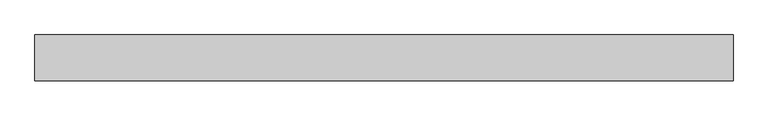
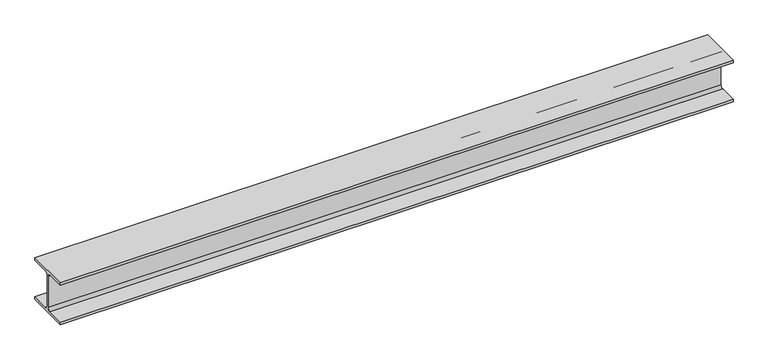
"""IFC4 building model written with IfcOpenShell, lengths in millimetres: beam geometry, 0912_Steel Framing_H-KSD3502 : H_SB_ASB_H-200x200x8x12."""

from ifc_helpers import new_model, si_unit, point, frame, frame_2d, origin, place, context, project, spatial, polyline, circle_curve, trimmed, segment, composite_curve, outline, extrude, source, transform, mapped, element, save


def beam_a4cbd311(model_context):
    return source(origin(), model_context, "Body", "SweptSolid", [
        extrude(outline(composite_curve([segment(polyline([(100.0, -88.0), (100.0, -100.0), (-100.0, -100.0), (-100.0, -88.0), (-17.0, -88.0)]), True, "CONTINUOUS"), segment(trimmed(circle_curve(frame_2d((-17.0, -75.0)), 13.0), [point((-17.0, -88.0))], [point((-4.0, -75.0))], True, "CARTESIAN"), True, "CONTINUOUS"), segment(polyline([(-4.0, -75.0), (-4.0, 75.0)]), True, "CONTINUOUS"), segment(trimmed(circle_curve(frame_2d((-17.0, 75.0)), 13.0), [point((-4.0, 75.0))], [point((-17.0, 88.0))], True, "CARTESIAN"), True, "CONTINUOUS"), segment(polyline([(-17.0, 88.0), (-100.0, 88.0), (-100.0, 100.0), (100.0, 100.0), (100.0, 88.0), (17.0, 88.0)]), True, "CONTINUOUS"), segment(trimmed(circle_curve(frame_2d((17.0, 75.0)), 13.0), [point((17.0, 88.0))], [point((4.0, 75.0))], True, "CARTESIAN"), True, "CONTINUOUS"), segment(polyline([(4.0, 75.0), (4.0, -75.0)]), True, "CONTINUOUS"), segment(trimmed(circle_curve(frame_2d((17.0, -75.0)), 13.0), [point((4.0, -75.0))], [point((17.0, -88.0))], True, "CARTESIAN"), True, "CONTINUOUS"), segment(polyline([(17.0, -88.0), (100.0, -88.0)]), True, "CONTINUOUS")], self_intersect=False)), frame((-1342.7433978, 0.0, 0.0), z_axis=(1.0, 0.0, 0.0), x_axis=(0.0, 1.0, 0.0)), (0.0, 0.0, 1.0), 3052.6875076),
    ])


if __name__ == "__main__":
    model = new_model("IFC4")
    model_context = context("Model", 3, world=origin())
    ifc_project = project(units=[si_unit("LENGTHUNIT", "METRE", prefix="MILLI")], contexts=[model_context])
    site = spatial("IfcSite", under=ifc_project)
    building = spatial("IfcBuilding", under=site)
    placement = place(None, origin())
    beam_shape = beam_a4cbd311(model_context)
    element("IfcBeam", 1, ObjectType="0912_Steel Framing_H-KSD3502 : H_SB_ASB_H-200x200x8x12", at=placement, inside=building, context=model_context, shape_type="MappedRepresentation", body=[
        mapped(beam_shape, transform((0.0, 0.0, 0.0), x_axis=(1.0, 0.0, 0.0), y_axis=(0.0, 1.0, 0.0), z_axis=(0.0, 0.0, 1.0))),
    ])
    save(model, "model.ifc")

# Revit data of these elements
# Type "0912_Steel Framing_H-KSD3502 : H_SB_ASB_H-200x200x8x12"
#   H_WM Code_1 = "S01AA002-00001 | Main Steel Structure Fabrication Work | Shelter/Building | Medium Steel - Standard (90KG/M>Weight≥30KG/M) | Material: (   )"
#   H_WM Code_2 = "S03AA028-00001 | Main Steel Structure Erection Work | Shelter/Building | Medium Steel (90KG/M>Weight≥30KG/M) | Material: (   )"
#   H_WM Code_3 = "S01AA010-00001 | Main Steel Structure Fabrication Work | Shelter/Building | Steel Painting/Coating | for Non-Fireproofed Steel Surface, Surface Preparation, Primer, Second & Final Coat | Material: (   )"
#   H_Q'ty Cal Type Tag = "SB-Q2"
#   Width = 20.0 cm
#   Web Thickness = 0.8 cm
#   Web Fillet = 1.3 cm
#   Warping Constant = 141000.0 cm⁶
#   W = 0
#   Torsional Moment of Inertia = 26.2485 cm⁴
#   Section Area = 63.53 cm²
#   Plastic Modulus weak axis = 244.0 cm³
#   Plastic Modulus strong axis = 525.0 cm³
#   Perimeter = 1.16 m²/m
#   Nominal Weight = 49.90 kgf/m
#   Moment of Inertia weak axis = 1600.00 cm⁴
#   Moment of Inertia strong axis = 4720.00 cm⁴
#   Height = 20.0 cm
#   Flange Thickness = 1.2 cm
#   Elastic Modulus weak axis = 160.0 cm³
#   Elastic Modulus strong axis = 472.0 cm³
#   Centroid Vertical = 10.0 cm
#   Centroid Horizontal = 10.0 cm
#   Ix = 47200000
#   Length [instance default] = 1.5240 m
#   Zx = 525000
#   b = 0.2000 m
#   h = 0.2000 m
#   r = 0.0130 m
#   s = 0.0080 m
#   t = 0.0120 m
#   A = 0.006353 m²
#   Structural Material [instance default] = Steel, 45-345
#   Assembly Code = ""
# Element 1 (IfcBeam, "0912_Steel Framing_H-KSD3502 : H_SB_ASB_H-200x200x8x12")
#   Structural Material = none
# Materials
#   "Steel, 45-345": class "Metal", colour RGB 189 187 185, transparency 0, Description = "Steel 345 MPa", Cost = 0
